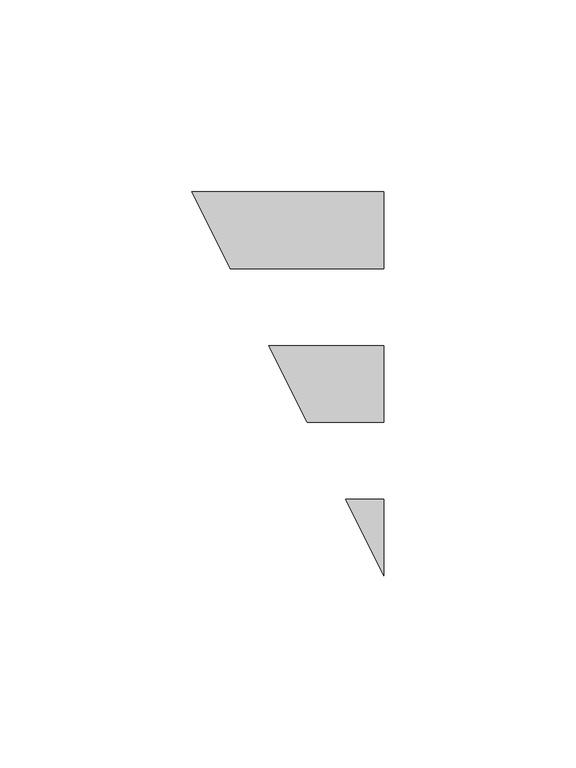
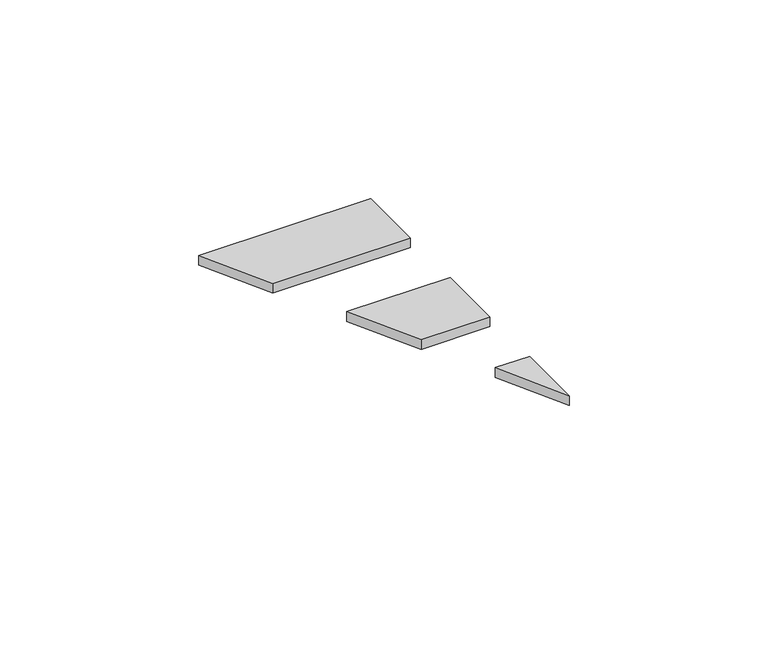
"""IFC4 building model written with IfcOpenShell, lengths in millimetres: proxy geometry, TSP Underfloor heating points : TSP Underfloor heating points."""

import ifcopenshell
import ifcopenshell.guid

model = None  # the IFC model being written
_history = None  # IfcOwnerHistory: only IFC2X3 demands one
_inside = {}  # id of a spatial element -> (the spatial element, [elements in it])
_under = {}  # id of a project, library or spatial element -> (it, [spatial elements below it])
_declared = {}  # id of a project -> (the project, [libraries it declares])
_typed = {}  # id of a type object -> (the type object, [elements of that type])
_made_of = {}  # id of a material, layer set ... -> (it, [elements and type objects made of it])


def new_model(schema):
    """Start an empty IFC model of exactly this schema.

    Asked for "IFC4X3", IfcOpenShell would pick the latest addendum, in which some entities
    have other attributes; the version numbers below select the first issue.
    IFC2X3 requires an IfcOwnerHistory on every rooted entity: one is made here for all.
    """
    global model, _history
    if schema == "IFC4X3":
        model = ifcopenshell.file(schema_version=(4, 3, 0, 0))
    else:
        model = ifcopenshell.file(schema=schema)
    _inside.clear()
    _under.clear()
    _declared.clear()
    _typed.clear()
    _made_of.clear()
    _history = None
    if model.schema == "IFC2X3":
        org = make("IfcOrganization", Name="unknown")
        user = make(
            "IfcPersonAndOrganization",
            ThePerson=make("IfcPerson", FamilyName="unknown"),
            TheOrganization=org,
        )
        app = make(
            "IfcApplication",
            ApplicationDeveloper=org,
            Version="unknown",
            ApplicationFullName="unknown",
            ApplicationIdentifier="unknown",
        )
        _history = make(
            "IfcOwnerHistory",
            OwningUser=user,
            OwningApplication=app,
            ChangeAction="ADDED",
            CreationDate=0,
        )
    return model


def make(cls, **values):
    """One entity of the class cls with the attributes given. An attribute that is None is left unset."""
    return model.create_entity(
        cls, **{name: value for name, value in values.items() if value is not None}
    )


def rooted(cls, **values):
    """An entity with a GlobalId (a new one), such as an element, a storey or a relation."""
    return make(cls, GlobalId=ifcopenshell.guid.new(), OwnerHistory=_history, **values)


def si_unit(unit_type, name, prefix=None):
    """IfcSIUnit, for example si_unit("LENGTHUNIT", "METRE", prefix="MILLI")."""
    return make("IfcSIUnit", UnitType=unit_type, Prefix=prefix, Name=name)


def assignment(units):
    """IfcUnitAssignment: the units of a project."""
    return None if units is None else make("IfcUnitAssignment", Units=units)


def point(xyz):
    """IfcCartesianPoint."""
    return None if xyz is None else make("IfcCartesianPoint", Coordinates=xyz)


def direction(xyz):
    """IfcDirection."""
    return None if xyz is None else make("IfcDirection", DirectionRatios=xyz)


def frame(location, z_axis=None, x_axis=None):
    """IfcAxis2Placement3D, a coordinate frame: its origin and axes. An axis left out is left unset."""
    return make(
        "IfcAxis2Placement3D",
        Location=point(location),
        Axis=direction(z_axis),
        RefDirection=direction(x_axis),
    )


def origin():
    """The frame at (0, 0, 0) with its axes left unset."""
    return frame((0.0, 0.0, 0.0))


def origin_with_axes():
    """The frame at (0, 0, 0) with the z axis (0, 0, 1) and the x axis (1, 0, 0) written out."""
    return frame((0.0, 0.0, 0.0), z_axis=(0.0, 0.0, 1.0), x_axis=(1.0, 0.0, 0.0))


def place(relative_to, where):
    """IfcLocalPlacement: puts the frame where relative to a parent placement (None: the world)."""
    return make(
        "IfcLocalPlacement", PlacementRelTo=relative_to, RelativePlacement=where
    )


def context(
    kind, dimensions, precision=None, world=None, true_north=None, identifier=None
):
    """IfcGeometricRepresentationContext, for example the 3D "Model" context."""
    return make(
        "IfcGeometricRepresentationContext",
        ContextIdentifier=identifier,
        ContextType=kind,
        CoordinateSpaceDimension=dimensions,
        Precision=precision,
        WorldCoordinateSystem=world,
        TrueNorth=true_north,
    )


def project(units=None, contexts=None):
    """IfcProject with its units and contexts."""
    return rooted(
        "IfcProject",
        Name="project",
        RepresentationContexts=contexts,
        UnitsInContext=assignment(units),
    )


def spatial(cls, under=None, at=None, **own):
    """A site, building, storey or space (cls), placed at a placement, below another one or the project."""
    s = rooted(cls, ObjectPlacement=at, **own)
    if under is not None:
        _under.setdefault(under.id(), (under, []))[1].append(s)
    return s


def polyline(points):
    """IfcPolyline through the points."""
    return make("IfcPolyline", Points=[point(p) for p in points])


def outline(outer, holes=None, kind="AREA"):
    """IfcArbitraryClosedProfileDef: a profile drawn as a closed curve; with holes, ...WithVoids."""
    if holes is None:
        return make("IfcArbitraryClosedProfileDef", ProfileType=kind, OuterCurve=outer)
    return make(
        "IfcArbitraryProfileDefWithVoids",
        ProfileType=kind,
        OuterCurve=outer,
        InnerCurves=holes,
    )


def extrude(swept, where, along, depth):
    """IfcExtrudedAreaSolid: the profile swept, set in the frame where, extruded along a direction by depth."""
    return make(
        "IfcExtrudedAreaSolid",
        SweptArea=swept,
        Position=where,
        ExtrudedDirection=direction(along),
        Depth=depth,
    )


def shape(context_of_items, identifier, shape_type, items):
    """IfcShapeRepresentation: the items that make up one representation, for example the "Body"."""
    return make(
        "IfcShapeRepresentation",
        ContextOfItems=context_of_items,
        RepresentationIdentifier=identifier,
        RepresentationType=shape_type,
        Items=items,
    )


def source(mapping_origin, context_of_items, identifier, shape_type, items):
    """IfcRepresentationMap: a shape defined once, which mapped items show again and again."""
    return make(
        "IfcRepresentationMap",
        MappingOrigin=mapping_origin,
        MappedRepresentation=shape(context_of_items, identifier, shape_type, items),
    )


def transform(
    local_origin,
    x_axis=None,
    y_axis=None,
    z_axis=None,
    scale=None,
    scale2=None,
    scale3=None,
    uniform=True,
):
    """IfcCartesianTransformationOperator3D, or its non-uniform kind. x_axis, y_axis, z_axis: its Axis1, 2, 3."""
    if uniform:
        return make(
            "IfcCartesianTransformationOperator3D",
            Axis1=direction(x_axis),
            Axis2=direction(y_axis),
            LocalOrigin=point(local_origin),
            Scale=scale,
            Axis3=direction(z_axis),
        )
    return make(
        "IfcCartesianTransformationOperator3DnonUniform",
        Axis1=direction(x_axis),
        Axis2=direction(y_axis),
        LocalOrigin=point(local_origin),
        Scale=scale,
        Axis3=direction(z_axis),
        Scale2=scale2,
        Scale3=scale3,
    )


def mapped(mapping_source, mapping_target):
    """IfcMappedItem: shows the shape of a source again, moved by a transform."""
    return make(
        "IfcMappedItem", MappingSource=mapping_source, MappingTarget=mapping_target
    )


def made_of(thing, what):
    """Note that an element or type object is made of a material, layer set ...; save() writes the relation."""
    if what is not None:
        _made_of.setdefault(what.id(), (what, []))[1].append(thing)
    return thing


def element(
    cls,
    number,
    at=None,
    inside=None,
    cuts=None,
    type_object=None,
    material=None,
    context=None,
    identifier="Body",
    shape_type=None,
    held_by="IfcProductDefinitionShape",
    body=None,
    shapes=None,
    **own,
):
    """One element of the class cls, such as IfcWall. Its Tag is "e" and its number.

    at: its placement. inside: the storey or other place that contains it. cuts: it is an
    opening in that element (IfcRelVoidsElement). A single representation is given by context,
    identifier, shape_type and body (its items); several are given by shapes. held_by: the class
    of the entity that holds the representations. save() writes the other relations.
    """
    e = rooted(cls, Tag="e%d" % number, ObjectPlacement=at, **own)
    if body is not None:
        shapes = [shape(context, identifier, shape_type, body)]
    if shapes is not None:
        e.Representation = make(held_by, Representations=shapes)
    if inside is not None:
        _inside.setdefault(inside.id(), (inside, []))[1].append(e)
    if cuts is not None:
        rooted(
            "IfcRelVoidsElement", RelatingBuildingElement=cuts, RelatedOpeningElement=e
        )
    if type_object is not None:
        _typed.setdefault(type_object.id(), (type_object, []))[1].append(e)
    return made_of(e, material)


def aggregate(whole, parts):
    """IfcRelAggregates: a whole, such as a stair, and the parts it consists of."""
    return rooted("IfcRelAggregates", RelatingObject=whole, RelatedObjects=parts)


def save(model, path):
    """Write the relations noted so far, then the file.

    IfcRelAggregates (storeys below a building ...), IfcRelContainedInSpatialStructure (elements
    in a storey), IfcRelDefinesByType, IfcRelAssociatesMaterial and IfcRelDeclares: one each for
    every whole, place, type object, material and project.
    """
    for whole, parts in _under.values():
        aggregate(whole, parts)
    for where, things in _inside.values():
        rooted(
            "IfcRelContainedInSpatialStructure",
            RelatedElements=things,
            RelatingStructure=where,
        )
    for kind, things in _typed.values():
        rooted("IfcRelDefinesByType", RelatedObjects=things, RelatingType=kind)
    for what, things in _made_of.values():
        rooted("IfcRelAssociatesMaterial", RelatedObjects=things, RelatingMaterial=what)
    for by, libraries in _declared.values():
        rooted("IfcRelDeclares", RelatingContext=by, RelatedDefinitions=libraries)
    model.write(path)


def electrical_fixtures_4ad4eb8e(model_context):
    return source(origin(), model_context, "Body", "SweptSolid", [
        extrude(outline(polyline([(0.0, -10.0), (-20.0, -10.0), (-30.0, 10.0), (0.0, 10.0), (0.0, -10.0)])), origin_with_axes(), (0.0, 0.0, 1.0), 3.0),
        extrude(outline(polyline([(-50.0, 50.0), (0.0, 50.0), (0.0, 30.0), (-40.0, 30.0), (-50.0, 50.0)])), origin_with_axes(), (0.0, 0.0, 1.0), 3.0),
        extrude(outline(polyline([(0.0, -30.0), (0.0, -50.0), (-10.0, -30.0), (0.0, -30.0)])), origin_with_axes(), (0.0, 0.0, 1.0), 3.0),
    ])


if __name__ == "__main__":
    model = new_model("IFC4")
    model_context = context("Model", 3, world=origin())
    ifc_project = project(units=[si_unit("LENGTHUNIT", "METRE", prefix="MILLI")], contexts=[model_context])
    site = spatial("IfcSite", under=ifc_project)
    building = spatial("IfcBuilding", under=site)
    placement = place(None, origin())
    electrical_fixtures_shape = electrical_fixtures_4ad4eb8e(model_context)
    element("IfcBuildingElementProxy", 1, Name="TSP Underfloor heating points : TSP Underfloor heating points", ObjectType="TSP Underfloor heating points : TSP Underfloor heating points", at=placement, inside=building, context=model_context, shape_type="MappedRepresentation", body=[
        mapped(electrical_fixtures_shape, transform((0.0, 0.0, 0.0), x_axis=(1.0, 0.0, 0.0), y_axis=(0.0, 1.0, 0.0), z_axis=(0.0, 0.0, 1.0))),
    ])
    save(model, "model.ifc")

# Revit data of these elements
# Type "TSP Underfloor heating points : TSP Underfloor heating points"
#   Model = "TSP_ELECUFHP"
#   Default Elevation = 0
# Element 1 (IfcBuildingElementProxy, "TSP Underfloor heating points : TSP Underfloor heating points")
#   Materials on its faces: "Plastic, Opaque Black"
# Materials
#   "Plastic, Opaque Black": class "Plastic", colour RGB 0 0 0, transparency 0.7, Description = "Plastic, generic, opaque black", Cost = 0
